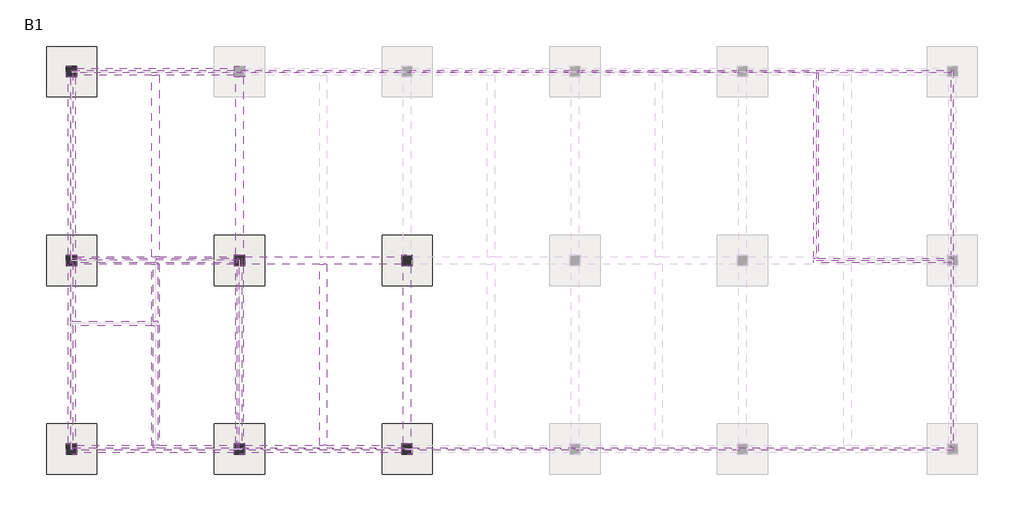
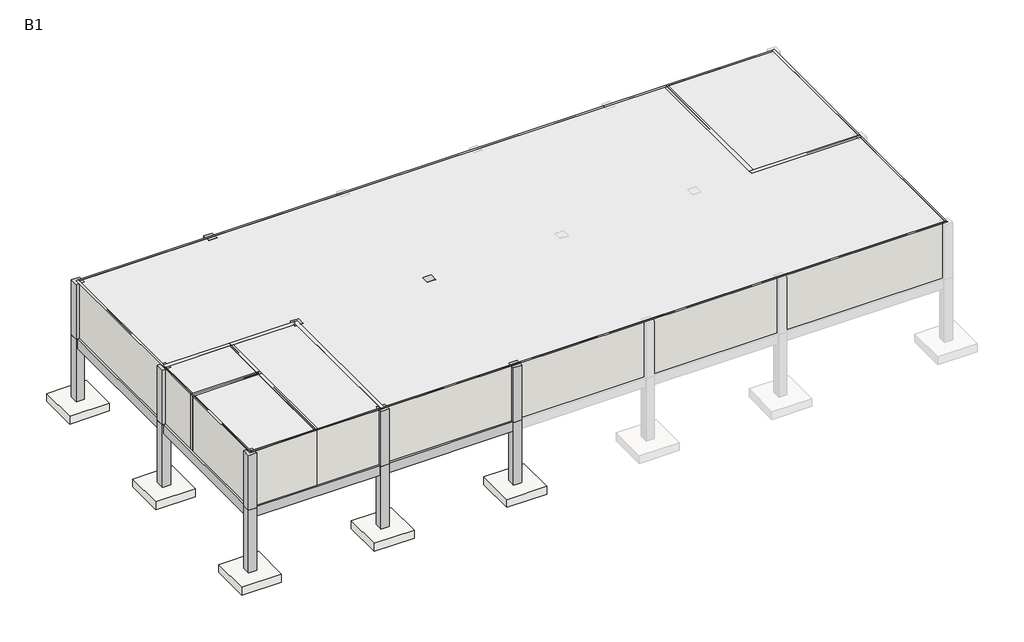
# One storey, part 1 of 2: 18 walls, 15 columns, 13 beams, 12 slabs.
# Revit data of these elements (continued)
# Elements 51, 54, 55, 56 (IfcWall, "WA221_Interior-Cement Block-190mm") (continued)
#   Materials on its faces: "Default Wall", "A04AS164-00002_Plastering_Int"
# Elements 52, 53, 58 (IfcWall, "WA221_Interior-Cement Block-190mm")
#   Top Offset = 0 mm
#   Base Offset = 0 mm
#   Unconnected Height = 3500 mm
#   wall height = 3500 mm
#   Phase Created = New Construction
#   Base Constraint = GF
#   Materials on its faces: "A04AS164-00002_Plastering_Int", "Default Wall", "A04AS164-00001_Plastering_Ext"
# Element 57 (IfcWall, "WA221_Interior-Cement Block-190mm")
#   Top Offset = 0 mm
#   Base Offset = 0 mm
#   Unconnected Height = 3500 mm
#   wall height = 3500 mm
#   Phase Created = New Construction
#   Base Constraint = GF
#   Materials on its faces: "Default Wall", "A04AS164-00002_Plastering_Int", "A04AS164-00001_Plastering_Ext"
# Materials
#   "콘크리트 - 현장타설 콘크리트": class "콘크리트", colour RGB 192 192 192, transparency 0
#   "A03AE056-00001_Bitumen/Bituminous/Asphalt Coating": class "Generic", colour RGB 17 17 17, transparency 0, Description = "Damp-proofing", W00) Work Master Code = "A03AE056-00001", W01) Work Master_Lv1 = "Concrete Work", W02) Work Master_Lv2 = "Concrete Protective Coating (U/G)", W03) Work Master_Spec.1 = "Bitumen/Bituminous/Asphalt Coating", Cost = 0
#   "A03AC035-00001_Form Work (3 times in use)_Flat": class "Wood", colour RGB 149 120 74, transparency 0, Description = "Plywood", W00) Work Master Code = "A03AC035-00001", W01) Work Master_Lv1 = "Concrete Work", W02) Work Master_Lv2 = "Substructure Work", W03) Work Master_Spec.1 = "Form Work (3 times in use)", W04) Work Master_Spec.2 = "Flat Form", W05) Work Master_Spec.3 = "Dressed Lumber, Plywood or Steel Form(Wood Planks are not Allowed) incl. Chamfer", Cost = 0
#   "A03AC032-00007_Structural Concrete_Type1_25MPa-30Mpa": class "Concrete", colour RGB 176 176 176, transparency 0, Keynote = "09910.A1", Description = "Reinf. Conc.", W00) Work Master Code = "A03AC032-00007", W01) Work Master_Lv1 = "Concrete Work", W02) Work Master_Lv2 = "Substructure Work", W03) Work Master_Spec.1 = "Structural Concrete", W04) Work Master_Spec.2 = "Cement Type-1", W05) Work Master_Spec.3 = "25MPa < F'c (Cylinder Strength) ≤ 30MPa", Cost = 0
#   "14200-030101_Concrete Pouring": class "Concrete", colour RGB 176 176 176, transparency 0, Description = "Reinf. Conc.", W00) Work Master Code = "14200-030101", W01) Work Master_Lv1 = "Concrete Work", W02) Work Master_Lv2 = "Building/Shelter Foundation Work", W03) Work Master_Spec.1 = "Concrete Pouring", W04) Work Master_Spec.2 = "F'c (Cylinder Strength) > 35MPa", W05) Work Master_Spec.3 = "Cement Type-1", Cost = 0
#   "A04AL081-00001_Skirt_Acrylic Emulsion Paint": class "Finish", colour RGB 128 128 64, transparency 0, Description = "Plastic", W00) Work Master Code = "A04AL081-00001", W01) Work Master_Lv1 = "Finishing Work", W02) Work Master_Lv2 = "Painting Work", W03) Work Master_Spec.1 = "Skirt Painting", W04) Work Master_Spec.2 = "Acrylic Emulsion Paint", W05) Work Master_Spec.3 = "100mm≤H<150mm", Cost = 0
#   "A04AL077-00001_Ext Wall Painting_Acrylic Emulsion Paint": class "Finish", colour RGB 128 128 64, transparency 0, Description = "Plastic", W00) Work Master Code = "A04AL077-00001", W01) Work Master_Lv1 = "Finishing Work", W02) Work Master_Lv2 = "Painting Work", W03) Work Master_Spec.1 = "External Wall Painting", W04) Work Master_Spec.2 = "Acrylic Emulsion Paint", Cost = 0
#   "A04AS164-00001_Plastering_Ext": class "Concrete", colour RGB 183 186 184, transparency 0, W00) Work Master Code = "A04AS164-00001", W01) Work Master_Lv1 = "Finishing Work", W02) Work Master_Lv2 = "Plastering Work", W03) Work Master_Spec.1 = "Plastering", W04) Work Master_Spec.2 = "for External Masonry Wall", Cost = 0
#   "A04AK073-00001_Concrete Brick_0.5B": class "Concrete", colour RGB 180 180 180, transparency 0, Description = "Conc. Block", W00) Work Master Code = "A04AK073-00001", W01) Work Master_Lv1 = "Finishing Work", W02) Work Master_Lv2 = "Masonry Work", W03) Work Master_Spec.1 = "Concrete Brick", W04) Work Master_Spec.2 = "[0.5B] w/ All Reinf.(Lath, Steel Tie, Anchor Bar, Mortar, ETC.), Filler, Sealant, Lintel/Sill for Opening, ETC.", Cost = 0
#   "A04AS164-00002_Plastering_Int": class "Concrete", colour RGB 183 186 184, transparency 0, Description = "LATEX PAINT ON THK.15 CEMENT PLASTER", W00) Work Master Code = "A04AS164-00002", W01) Work Master_Lv1 = "Finishing Work", W02) Work Master_Lv2 = "Plastering Work", W03) Work Master_Spec.1 = "Plastering", W04) Work Master_Spec.2 = "for Internal Masonry Wall", Cost = 0
#   "A04AL078-00002_Int Wall Painting_Water Emulsion Paint": class "Finish", colour RGB 128 128 64, transparency 0, Description = "Plastic", W00) Work Master Code = "A04AL078-00002", W01) Work Master_Lv1 = "Finishing Work", W02) Work Master_Lv2 = "Painting Work", W03) Work Master_Spec.1 = "Internal Wall Painting", W04) Work Master_Spec.2 = "Water Emulsion Paint", Cost = 0
#   "A04AK069-00002_Reinforced Concrete Block_THK 100-200mm": class "Concrete", colour RGB 180 180 180, transparency 0, Description = "Conc. Block", W00) Work Master Code = "A04AK069-00002", W01) Work Master_Lv1 = "Finishing Work", W02) Work Master_Lv2 = "Masonry Work", W03) Work Master_Spec.1 = "Reinforced Concrete Block", W04) Work Master_Spec.2 = "w/ All Reinf.(Lath, Steel Tie, Anchor Bar, Mortar, ETC.), Filler, Sealant, Lintel/Sill for Opening, ETC.", W05) Work Master_Spec.3 = "100mm<THK≤200mm", Cost = 0
#   "Default Wall": class "Miscellaneous", colour RGB 80 80 80, transparency 0
# Room at (84209.652, 177423.861) mm, phase "New Construction", upper offset 3500 mm, lower offset 0 mm
#   Department = "EL"
#   Base Finish = ""
#   Ceiling Finish = "CL2"
#   Wall Finish = "IW2"
#   Floor Finish = "FL7"
#   Number = "0.0"
#   Name = "Battery Room"
#   Interior Finish = "IW2..N/A..N/A,,N/A..N/A,,FL7..N/A,,CL2..N/A"
#   Exterior Finish = "N/A..N/A,,EW2..N/A..N/A"
# Room at (51459.652, 168423.861) mm, phase "New Construction", upper offset 3500 mm, lower offset 0 mm
#   Department = "AR"
#   Base Finish = "WK3"
#   Ceiling Finish = ""
#   Wall Finish = "IW5"
#   Floor Finish = "FL2"
#   Number = "0.1"
#   Name = "Lobby"
#   Interior Finish = "IW5..N/A..N/A,,WK3..N/A,,FL2..N/A,,N/A..N/A"
#   Exterior Finish = "N/A..N/A,,EW2..N/A..N/A"
# Room at (66459.652, 172923.861) mm, phase "New Construction", upper offset 3500 mm, lower offset 0 mm
#   Department = "EL"
#   Base Finish = "WK1"
#   Ceiling Finish = "CL1"
#   Wall Finish = "IW5,IW2"
#   Floor Finish = "FL1"
#   Number = "0.2"
#   Name = "Cable Room"
#   Interior Finish = "IW5..IW2..N/A,,WK1..N/A,,FL1..N/A,,CL1..N/A"
#   Exterior Finish = "N/A..N/A,,EW1..EW2..N/A"
# Room at (47459.652, 166923.861) mm, phase "New Construction", upper offset 3500 mm, lower offset 0 mm
#   Department = "PATHV1"
#   Base Finish = "WK3"
#   Ceiling Finish = "CL1"
#   Wall Finish = "IW5"
#   Floor Finish = "FL2"
#   Number = "0.3"
#   Name = "Stairway"
#   Interior Finish = "IW5..N/A..N/A,,WK3..N/A,,FL2..N/A,,CL1..N/A"
#   Exterior Finish = "N/A..N/A,,EW2..N/A..N/A"
# Room at (47459.652, 171423.861) mm, phase "New Construction", upper offset 3500 mm, lower offset 0 mm
#   Department = "AR"
#   Base Finish = ""
#   Ceiling Finish = "CL3"
#   Wall Finish = ""
#   Floor Finish = ""
#   Number = "0.4"
#   Name = "Elevator"
#   Interior Finish = "N/A..N/A..N/A,,N/A..N/A,,,,CL3..N/A"
#   Exterior Finish = "N/A..N/A,,EW2..N/A..N/A"
